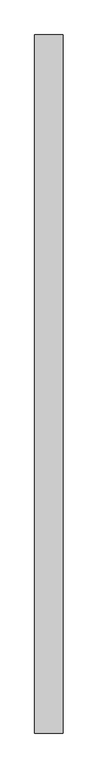
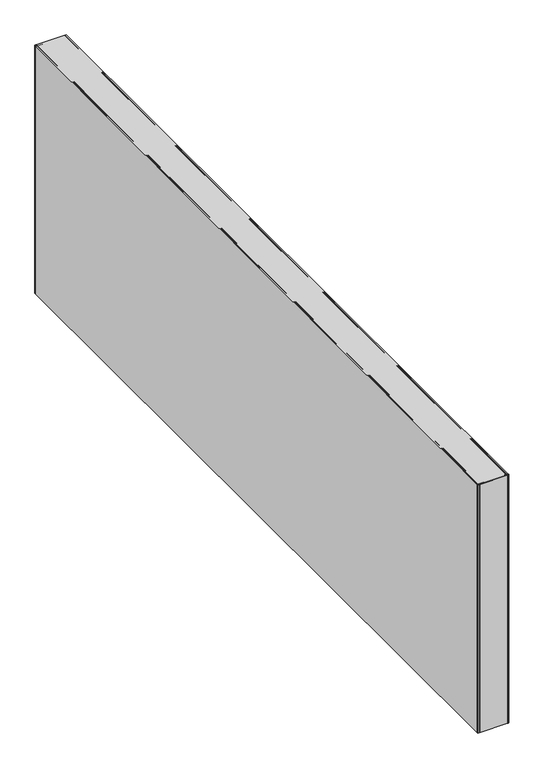
"""IFC4 building model written with IfcOpenShell, lengths in millimetres: beam geometry, LF02ZBK001_DIKE WALL_RC : Dike_Thk.250_EW3."""

from ifc_helpers import new_model, si_unit, origin, origin_with_axes, place, context, project, spatial, polyline, outline, extrude, source, transform, mapped, element, save


def beam_d786ea5f(model_context):
    return source(origin(), model_context, "Body", "SweptSolid", [
        extrude(outline(polyline([(125.0, -3072.5), (-125.0, -3072.5), (-125.0, 3072.5), (125.0, 3072.5), (125.0, -3072.5)])), origin_with_axes(), (0.0, 0.0, 1.0), 2100.0),
        extrude(outline(polyline([(-125.0, -3057.5), (-125.0, -3056.5), (125.0, -3056.5), (125.0, -3057.5), (-125.0, -3057.5)])), origin_with_axes(), (0.0, 0.0, 1.0), 2100.0),
        extrude(outline(polyline([(-125.0, -3062.5), (-125.0, -3061.5), (125.0, -3061.5), (125.0, -3062.5), (-125.0, -3062.5)])), origin_with_axes(), (0.0, 0.0, 1.0), 2100.0),
        extrude(outline(polyline([(-125.0, -3067.5), (-125.0, -3066.5), (125.0, -3066.5), (125.0, -3067.5), (-125.0, -3067.5)])), origin_with_axes(), (0.0, 0.0, 1.0), 2100.0),
        extrude(outline(polyline([(-125.0, 3057.5), (125.0, 3057.5), (125.0, 3056.5), (-125.0, 3056.5), (-125.0, 3057.5)])), origin_with_axes(), (0.0, 0.0, 1.0), 2100.0),
        extrude(outline(polyline([(-125.0, 3062.5), (125.0, 3062.5), (125.0, 3061.5), (-125.0, 3061.5), (-125.0, 3062.5)])), origin_with_axes(), (0.0, 0.0, 1.0), 2100.0),
        extrude(outline(polyline([(-125.0, 3067.5), (125.0, 3067.5), (125.0, 3066.5), (-125.0, 3066.5), (-125.0, 3067.5)])), origin_with_axes(), (0.0, 0.0, 1.0), 2100.0),
        extrude(outline(polyline([(109.0, 3072.5), (110.0, 3072.5), (110.0, -3072.5), (109.0, -3072.5), (109.0, 3072.5)])), origin_with_axes(), (0.0, 0.0, 1.0), 2100.0),
        extrude(outline(polyline([(114.0, 3072.5), (115.0, 3072.5), (115.0, -3072.5), (114.0, -3072.5), (114.0, 3072.5)])), origin_with_axes(), (0.0, 0.0, 1.0), 2100.0),
        extrude(outline(polyline([(119.0, 3072.5), (120.0, 3072.5), (120.0, -3072.5), (119.0, -3072.5), (119.0, 3072.5)])), origin_with_axes(), (0.0, 0.0, 1.0), 2100.0),
        extrude(outline(polyline([(-109.0, 3072.5), (-109.0, -3072.5), (-110.0, -3072.5), (-110.0, 3072.5), (-109.0, 3072.5)])), origin_with_axes(), (0.0, 0.0, 1.0), 2100.0),
        extrude(outline(polyline([(-114.0, 3072.5), (-114.0, -3072.5), (-115.0, -3072.5), (-115.0, 3072.5), (-114.0, 3072.5)])), origin_with_axes(), (0.0, 0.0, 1.0), 2100.0),
        extrude(outline(polyline([(-119.0, 3072.5), (-119.0, -3072.5), (-120.0, -3072.5), (-120.0, 3072.5), (-119.0, 3072.5)])), origin_with_axes(), (0.0, 0.0, 1.0), 2100.0),
    ])


if __name__ == "__main__":
    model = new_model("IFC4")
    model_context = context("Model", 3, world=origin())
    ifc_project = project(units=[si_unit("LENGTHUNIT", "METRE", prefix="MILLI")], contexts=[model_context])
    site = spatial("IfcSite", under=ifc_project)
    building = spatial("IfcBuilding", under=site)
    placement = place(None, origin())
    beam_shape = beam_d786ea5f(model_context)
    element("IfcBeam", 1, ObjectType="LF02ZBK001_DIKE WALL_RC : Dike_Thk.250_EW3", at=placement, inside=building, context=model_context, shape_type="MappedRepresentation", body=[
        mapped(beam_shape, transform((0.0, 0.0, 0.0), x_axis=(1.0, 0.0, 0.0), y_axis=(0.0, 1.0, 0.0), z_axis=(0.0, 0.0, 1.0))),
    ])
    save(model, "model.ifc")

# Revit data of these elements
# Type "LF02ZBK001_DIKE WALL_RC : Dike_Thk.250_EW3"
#   Dike_thk = 250 mm
#   Dike_Length [instance default] = 3000 mm
#   Dike_Hight = 2100 mm
#   c2_visible = yes
#   c3_material [instance default] = none
#   c2_material 3 [instance default] = none
#   c2_material 2 [instance default] = none
#   c2_material 1 [instance default] = none
#   c1_material [instance default] = none
#   Default Elevation = 0
# Element 1 (IfcBeam, "LF02ZBK001_DIKE WALL_RC : Dike_Thk.250_EW3")
#   Dike_Length = 6145 mm
